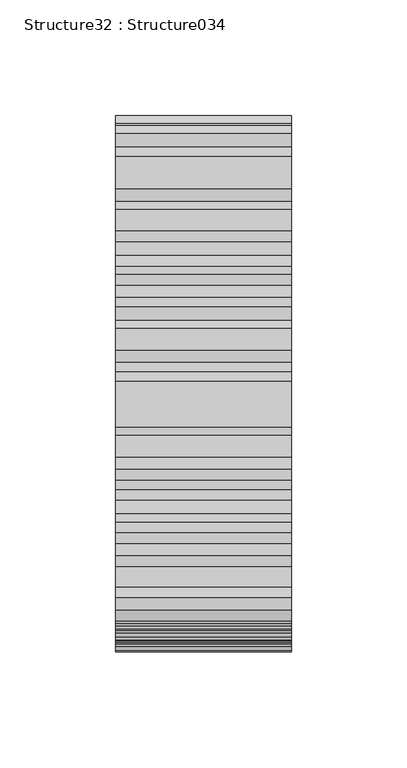
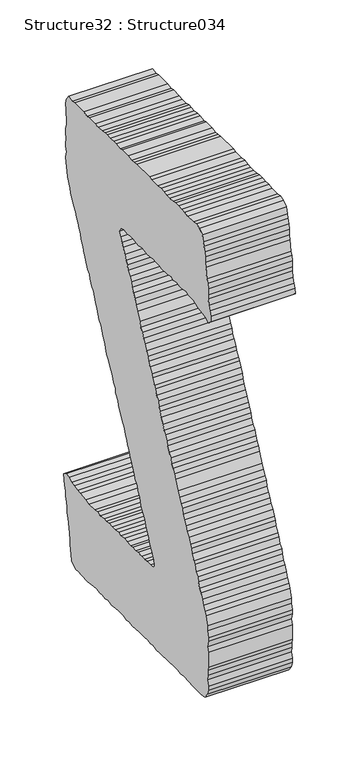
"""IFC4 building model written with IfcOpenShell, lengths in millimetres: proxy geometry, Structure32 : Structure034."""

from ifc_helpers import new_model, si_unit, frame, origin, place, context, project, spatial, polyline, outline, extrude, source, transform, mapped, element, save


def structure32_structure034_fc4fab0b(model_context):
    return source(origin(), model_context, "Body", "SweptSolid", [
        extrude(outline(polyline([(253013.5433895, 3631.3410106), (253012.952895, 3626.0554434), (253011.7767199, 3621.3732075), (253010.6021494, 3616.69739), (253010.6021494, 3612.0135494), (253008.8515259, 3606.7295868), (253008.2594269, 3602.6298224), (253007.6785601, 3597.3538828), (253006.5007804, 3592.6700423), (253005.9263319, 3589.1527492), (253004.7517615, 3584.4689087), (253004.161267, 3579.7690221), (253003.577191, 3573.9266571), (253003.577191, 3569.8268927), (253002.4090389, 3565.1254015), (253001.8281721, 3561.025637), (253000.6423693, 3555.1848766), (252994.2095099, 3551.0658569), (252990.1001178, 3551.6675836), (252986.0003533, 3551.0658569), (252975.4581018, 3551.0658569), (252966.0743747, 3552.242032), (252961.9730056, 3552.242032), (252956.7066936, 3551.6675836), (252952.0132255, 3552.242032), (252948.5055601, 3551.0658569), (252943.8120919, 3552.242032), (252937.9536809, 3551.0658569), (252927.9874824, 3552.242032), (252919.2022728, 3552.242032), (252914.5200368, 3551.0658569), (252910.4090401, 3552.242032), (252905.1347052, 3551.0658569), (252899.8683932, 3551.0658569), (252895.174925, 3551.6675836), (252886.4009477, 3551.6675836), (252881.1234035, 3552.242032), (252877.015616, 3551.0658569), (252872.9158515, 3552.242032), (252867.0654635, 3551.0658569), (252862.3719953, 3551.6675836), (252857.0880327, 3551.0658569), (252852.4138198, 3551.6675836), (252834.8289592, 3551.6675836), (252828.9689436, 3551.0658569), (252825.4612781, 3551.6675836), (252815.493475, 3551.6675836), (252810.8112391, 3551.0658569), (252797.3341659, 3551.0658569), (252791.4757549, 3551.6675836), (252787.3743858, 3556.9258725), (252786.1998153, 3561.6257591), (252786.1998153, 3565.7094775), (252787.3743858, 3570.9854171), (252786.7822868, 3575.6853037), (252786.7822868, 3580.3691442), (252786.1998153, 3583.8864372), (252786.1998153, 3597.9540049), (252787.3743858, 3602.6298224), (252786.1998153, 3608.4705827), (252786.1998153, 3612.0135494), (252787.3743858, 3617.8559144), (252787.3743858, 3622.555801), (252789.7171084, 3630.7392839), (252791.4757549, 3634.2822506), (252793.8168729, 3638.3563415), (252795.5755194, 3643.0578326), (252797.3341659, 3648.3161216), (252799.6849115, 3651.2589662), (252801.435535, 3656.5429288), (252802.6101055, 3660.6250426), (252805.5352995, 3663.5598643), (252807.3003644, 3669.4262983), (252808.4588889, 3672.3691429), (252811.9761819, 3677.0449604), (252812.568281, 3681.7271964), (252814.3269275, 3684.6443673), (252816.6696501, 3689.9540036), (252819.5932395, 3694.029699), (252821.351886, 3698.1294635), (252823.6946086, 3702.229228), (252826.0453542, 3706.3289925), (252826.618198, 3711.6145597), (252828.9689436, 3714.5301261), (252831.3116661, 3719.2316172), (252833.6624117, 3723.9154578), (252837.7541532, 3732.7167134), (252839.5224273, 3736.7988273), (252841.2810739, 3740.9162424), (252843.6205872, 3743.8414364), (252844.7967623, 3749.117376), (252847.7203517, 3752.6170184), (252850.0630743, 3757.3185096), (252851.2376447, 3761.418274), (252853.5803673, 3765.5019925), (252855.3390138, 3769.0176809), (252857.0880327, 3773.7015215), (252860.032482, 3778.4046172), (252861.7815009, 3783.0868532), (252863.5481704, 3786.6298199), (252864.7050903, 3791.3056374), (252867.0654635, 3795.4037973), (252869.3985584, 3800.0876378), (252870.5731289, 3803.0064134), (252874.090422, 3807.714323), (252874.682521, 3811.2043377), (252877.6061104, 3816.4883003), (252879.94081, 3820.015221), (252881.1234035, 3824.1149855), (252882.8756316, 3828.2163546), (252885.8088486, 3833.4730389), (252887.5578675, 3837.6000817), (252889.3245371, 3842.2758992), (252892.2513357, 3845.1914656), (252893.4259061, 3850.4754282), (252897.5352983, 3857.5019912), (252899.8683932, 3862.2018778), (252901.0429637, 3867.4601667), (252903.3856863, 3871.5599312), (252906.3092756, 3875.0772243), (252906.9013747, 3879.7610648), (252909.2440973, 3883.8881076), (252912.1773143, 3887.9621984), (252912.7517627, 3892.6636896), (252915.1025083, 3895.5888836), (252916.8611548, 3900.2887701), (252919.7943718, 3904.9645876), (252921.5433907, 3909.0627475), (252923.8957409, 3912.5896682), (252926.2368589, 3916.6653636), (252923.3116649, 3921.3748778), (252918.6198013, 3922.5494483), (252913.3454664, 3921.3748778), (252908.6600212, 3922.5494483), (252904.5602567, 3922.5494483), (252899.8683932, 3921.3748778), (252895.7670241, 3921.3748778), (252890.4926891, 3922.5494483), (252886.9737915, 3921.9733953), (252882.2995786, 3921.3748778), (252877.015616, 3921.3748778), (252872.9158515, 3922.5494483), (252868.8144824, 3921.9733953), (252862.9560714, 3921.9733953), (252859.448406, 3921.3748778), (252849.4709752, 3921.3748778), (252844.2126863, 3922.5494483), (252841.2810739, 3921.3748778), (252836.0035297, 3922.5494483), (252831.3116661, 3921.3748778), (252827.210297, 3921.3748778), (252821.351886, 3922.5494483), (252817.2521215, 3921.3748778), (252809.0525926, 3921.3748778), (252803.1925769, 3919.0321552), (252799.0928125, 3917.8479571), (252794.3993443, 3917.2735087), (252790.3011844, 3916.6653636), (252785.6077163, 3914.3499193), (252781.5063472, 3917.8479571), (252782.1000508, 3922.5494483), (252783.8570928, 3926.6492128), (252785.0316633, 3931.3346579), (252785.6077163, 3937.1930689), (252786.1998153, 3940.718385), (252786.1998153, 3946.5511223), (252786.7822868, 3951.2606365), (252787.9584619, 3954.7506513), (252789.7171084, 3964.7361051), (252790.8820512, 3968.8198235), (252790.8820512, 3974.1214368), (252791.4757549, 3978.8036727), (252792.6406978, 3983.4794902), (252793.8168729, 3987.0048063), (252794.9914434, 3992.8375436), (252799.6849115, 3996.390138), (252804.9512235, 3997.5486624), (252809.6334594, 3996.390138), (252818.4282966, 3996.390138), (252823.1105325, 3997.5486624), (252828.3848675, 3996.9645864), (252833.0783357, 3997.5486624), (252837.7541532, 3997.5486624), (252841.2810739, 3996.9645864), (252847.1378803, 3996.390138), (252851.8313484, 3996.390138), (252855.9311129, 3996.9645864), (252860.6053258, 3997.5486624), (252865.890893, 3996.9645864), (252875.258574, 3996.9645864), (252878.7838901, 3997.5486624), (252898.6922181, 3997.5486624), (252902.7919826, 3996.9645864), (252906.9013747, 3996.390138), (252912.1773143, 3997.5486624), (252921.5433907, 3997.5486624), (252925.0606838, 3996.390138), (252930.9287224, 3997.5486624), (252935.0300915, 3997.5486624), (252940.2947989, 3996.9645864), (252944.988267, 3997.5486624), (252948.5055601, 3997.5486624), (252953.187796, 3996.390138), (252959.0478116, 3996.390138), (252963.7412798, 3996.9645864), (252973.1073562, 3996.9645864), (252976.6150216, 3996.390138), (252981.8989842, 3997.5486624), (252995.9601334, 3997.5486624), (253000.0598979, 3996.390138), (253005.9263319, 3997.5486624), (253009.4452296, 3992.2614906), (253010.0260964, 3988.1633307), (253009.4452296, 3982.8793681), (253009.4452296, 3978.8036727), (253008.8515259, 3974.1214368), (253008.8515259, 3968.8198235), (253010.0260964, 3964.7361051), (253010.0260964, 3960.0602876), (253009.4452296, 3954.7506513), (253010.0260964, 3950.0940891), (253010.0260964, 3947.1496398), (253008.8515259, 3942.4770315), (253010.0260964, 3937.1930689), (253009.4452296, 3931.9058971), (253008.8515259, 3928.4158823), (253007.094484, 3919.6066036), (253002.9850919, 3911.4054701), (253002.4090389, 3906.7328618), (252999.4758219, 3901.44569), (252997.7187799, 3897.9476522), (252994.7919813, 3893.822214), (252993.0253118, 3889.7208449), (252990.6938215, 3885.6210804), (252989.5160418, 3880.9452629), (252986.5924524, 3877.4456205), (252986.0003533, 3872.745734), (252983.0767639, 3867.4601667), (252981.8989842, 3863.9332461), (252979.5578663, 3859.2606378), (252977.7895921, 3855.7353217), (252975.4581018, 3850.4754282), (252972.5232802, 3847.5598618), (252971.9392041, 3843.432819), (252969.5900631, 3838.1761347), (252966.6648691, 3834.6588416), (252964.9062226, 3830.5574726), (252963.1475761, 3825.849563), (252960.8048535, 3821.1737455), (252957.8732411, 3812.3901405), (252954.3559481, 3809.4729695), (252953.187796, 3804.7730829), (252951.4291495, 3800.6717138), (252948.5055601, 3795.4037973), (252947.3309896, 3791.8865042), (252945.5707384, 3787.2042683), (252942.6375214, 3783.0868532), (252941.4725786, 3779.5872107), (252939.121833, 3775.4874463), (252936.7791104, 3771.3860772), (252935.0300915, 3766.684586), (252932.0968745, 3762.5848215), (252931.5031708, 3758.485057), (252927.9874824, 3753.2171405), (252926.8193303, 3749.117376), (252924.479817, 3744.9999608), (252922.1370944, 3740.3161203), (252920.3688202, 3736.2163558), (252918.0357253, 3732.7167134), (252916.2770788, 3727.4311462), (252913.9263332, 3723.3313817), (252912.7517627, 3720.4158154), (252911.0027438, 3716.2887726), (252908.6600212, 3710.4560353), (252905.7268042, 3706.3289925), (252901.6270397, 3698.1294635), (252901.0429637, 3694.6298211), (252897.5352983, 3689.9540036), (252896.3511001, 3685.8285655), (252893.4259061, 3681.7271964), (252892.8418301, 3677.0449604), (252891.073556, 3672.9435914), (252885.8088486, 3665.3265338), (252884.0502021, 3660.0682449), (252881.7074795, 3655.3587307), (252879.3583385, 3651.2589662), (252878.7838901, 3647.1575971), (252875.258574, 3642.4833842), (252873.5079505, 3639.5405396), (252871.741281, 3634.2822506), (252870.5731289, 3630.7392839), (252871.741281, 3627.2396415), (252877.015616, 3626.6571701), (252882.2995786, 3627.2396415), (252886.4009477, 3626.6571701), (252891.073556, 3626.6571701), (252896.3511001, 3627.2396415), (252900.4588877, 3626.0554434), (252905.1347052, 3626.6571701), (252908.6600212, 3626.0554434), (252913.9263332, 3626.6571701), (252918.0357253, 3627.2396415), (252923.8957409, 3626.0554434), (252927.4114294, 3627.2396415), (252932.6777413, 3626.6571701), (252937.3712095, 3626.6571701), (252942.0534454, 3627.2396415), (252946.7388905, 3626.0554434), (252950.254579, 3626.6571701), (252956.1226176, 3626.0554434), (252960.2239867, 3627.2396415), (252964.9062226, 3626.0554434), (252974.2819267, 3626.0554434), (252978.9753948, 3627.2396415), (252987.7493722, 3628.4158166), (252991.2746883, 3628.998288), (252997.1347039, 3629.5984101), (253000.6423693, 3630.7392839), (253004.7517615, 3633.0980525), (253009.4452296, 3633.6821286), (253013.5433895, 3631.3410106)])), frame((-38594.2176606, 0.0, 0.0), z_axis=(1.0, 0.0, 0.0), x_axis=(0.0, 1.0, 0.0)), (0.0, 0.0, 1.0), 76.2),
    ])


if __name__ == "__main__":
    model = new_model("IFC4")
    model_context = context("Model", 3, world=origin())
    ifc_project = project(units=[si_unit("LENGTHUNIT", "METRE", prefix="MILLI")], contexts=[model_context])
    site = spatial("IfcSite", under=ifc_project)
    building = spatial("IfcBuilding", under=site)
    placement = place(None, origin())
    structure32_structure034_shape = structure32_structure034_fc4fab0b(model_context)
    element("IfcBuildingElementProxy", 1, Name="Structure32 : Structure034", ObjectType="Structure32 : Structure034", at=placement, inside=building, context=model_context, shape_type="MappedRepresentation", body=[
        mapped(structure32_structure034_shape, transform((0.0, 0.0, 0.0), x_axis=(1.0, 0.0, 0.0), y_axis=(0.0, 1.0, 0.0), z_axis=(0.0, 0.0, 1.0))),
    ])
    save(model, "model.ifc")

# Revit data of these elements
# Type "Structure32 : Structure034"
#   NameOverride = "Structure034"
# Element 1 (IfcBuildingElementProxy, "Structure32 : Structure034")
#   Materials on its faces: "BRUSHED ALUM. LETTERING"
# Materials
#   "BRUSHED ALUM. LETTERING": class "Unassigned", colour RGB 169 181 186, transparency 0, Cost = 0
